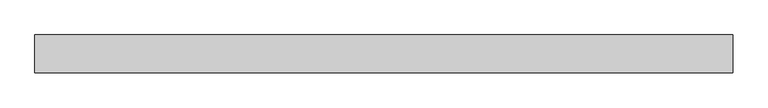
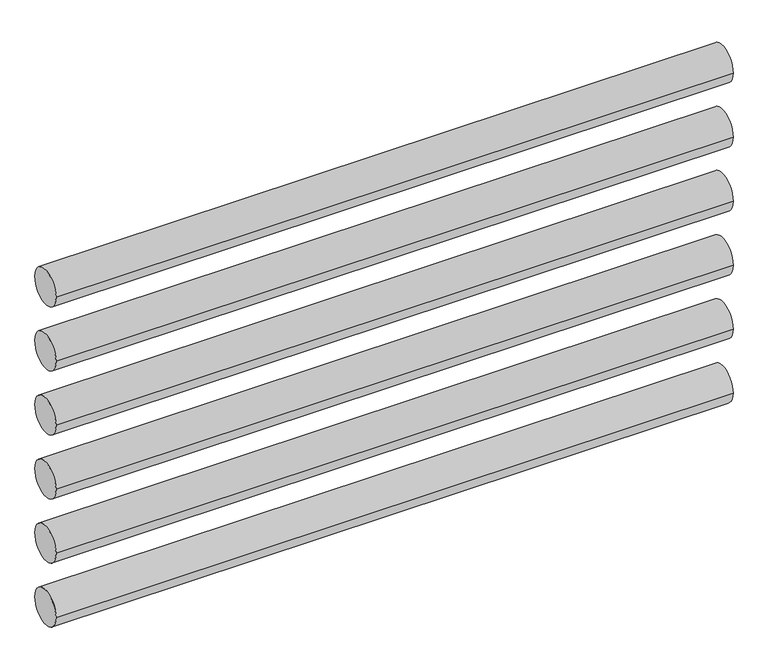
"""IFC4 building model written with IfcOpenShell, lengths in millimetres: proxy geometry, Газпремиум_Регистр : РГТ-1-108х3-2м-6."""

from ifc_helpers import new_model, si_unit, point, frame, frame_2d, origin, place, context, project, spatial, circle_curve, trimmed, segment, composite_curve, outline, extrude, source, transform, mapped, element, save


def mechanical_equipment_f739d76b(model_context):
    return source(origin(), model_context, "Body", "SweptSolid", [
        extrude(outline(composite_curve([segment(trimmed(circle_curve(frame_2d((0.0, 1054.0)), 54.0), [point((-54.0, 1054.0))], [point((54.0, 1054.0))], False, "CARTESIAN"), True, "CONTINUOUS"), segment(trimmed(circle_curve(frame_2d((0.0, 1054.0)), 54.0), [point((54.0, 1054.0))], [point((-54.0, 1054.0))], False, "CARTESIAN"), True, "CONTINUOUS")], self_intersect=False)), frame((-184.1719207, 0.0, 0.0), z_axis=(1.0, 0.0, 0.0), x_axis=(0.0, 1.0, 0.0)), (0.0, 0.0, 1.0), 2000.0),
        extrude(outline(composite_curve([segment(trimmed(circle_curve(frame_2d((0.0, 854.0)), 54.0), [point((-54.0, 854.0))], [point((54.0, 854.0))], False, "CARTESIAN"), True, "CONTINUOUS"), segment(trimmed(circle_curve(frame_2d((0.0, 854.0)), 54.0), [point((54.0, 854.0))], [point((-54.0, 854.0))], False, "CARTESIAN"), True, "CONTINUOUS")], self_intersect=False)), frame((-184.1719207, 0.0, 0.0), z_axis=(1.0, 0.0, 0.0), x_axis=(0.0, 1.0, 0.0)), (0.0, 0.0, 1.0), 2000.0),
        extrude(outline(composite_curve([segment(trimmed(circle_curve(frame_2d((0.0, 654.0)), 54.0), [point((-54.0, 654.0))], [point((54.0, 654.0))], False, "CARTESIAN"), True, "CONTINUOUS"), segment(trimmed(circle_curve(frame_2d((0.0, 654.0)), 54.0), [point((54.0, 654.0))], [point((-54.0, 654.0))], False, "CARTESIAN"), True, "CONTINUOUS")], self_intersect=False)), frame((-184.1719207, 0.0, 0.0), z_axis=(1.0, 0.0, 0.0), x_axis=(0.0, 1.0, 0.0)), (0.0, 0.0, 1.0), 2000.0),
        extrude(outline(composite_curve([segment(trimmed(circle_curve(frame_2d((0.0, 454.0)), 54.0), [point((-54.0, 454.0))], [point((54.0, 454.0))], False, "CARTESIAN"), True, "CONTINUOUS"), segment(trimmed(circle_curve(frame_2d((0.0, 454.0)), 54.0), [point((54.0, 454.0))], [point((-54.0, 454.0))], False, "CARTESIAN"), True, "CONTINUOUS")], self_intersect=False)), frame((-184.1719207, 0.0, 0.0), z_axis=(1.0, 0.0, 0.0), x_axis=(0.0, 1.0, 0.0)), (0.0, 0.0, 1.0), 2000.0),
        extrude(outline(composite_curve([segment(trimmed(circle_curve(frame_2d((0.0, 254.0)), 54.0), [point((-54.0, 254.0))], [point((54.0, 254.0))], False, "CARTESIAN"), True, "CONTINUOUS"), segment(trimmed(circle_curve(frame_2d((0.0, 254.0)), 54.0), [point((54.0, 254.0))], [point((-54.0, 254.0))], False, "CARTESIAN"), True, "CONTINUOUS")], self_intersect=False)), frame((-184.1719207, 0.0, 0.0), z_axis=(1.0, 0.0, 0.0), x_axis=(0.0, 1.0, 0.0)), (0.0, 0.0, 1.0), 2000.0),
        extrude(outline(composite_curve([segment(trimmed(circle_curve(frame_2d((0.0, 54.0)), 54.0), [point((-54.0, 54.0))], [point((54.0, 54.0))], False, "CARTESIAN"), True, "CONTINUOUS"), segment(trimmed(circle_curve(frame_2d((0.0, 54.0)), 54.0), [point((54.0, 54.0))], [point((-54.0, 54.0))], False, "CARTESIAN"), True, "CONTINUOUS")], self_intersect=False)), frame((-184.1719207, 0.0, 0.0), z_axis=(1.0, 0.0, 0.0), x_axis=(0.0, 1.0, 0.0)), (0.0, 0.0, 1.0), 2000.0),
    ])


if __name__ == "__main__":
    model = new_model("IFC4")
    model_context = context("Model", 3, world=origin())
    ifc_project = project(units=[si_unit("LENGTHUNIT", "METRE", prefix="MILLI")], contexts=[model_context])
    site = spatial("IfcSite", under=ifc_project)
    building = spatial("IfcBuilding", under=site)
    placement = place(None, origin())
    mechanical_equipment_shape = mechanical_equipment_f739d76b(model_context)
    element("IfcBuildingElementProxy", 1, Name="Газпремиум_Регистр : РГТ-1-108х3-2м-6", ObjectType="Газпремиум_Регистр : РГТ-1-108х3-2м-6", at=placement, inside=building, context=model_context, shape_type="MappedRepresentation", body=[
        mapped(mechanical_equipment_shape, transform((0.0, 0.0, 0.0), x_axis=(1.0, 0.0, 0.0), y_axis=(0.0, 1.0, 0.0), z_axis=(0.0, 0.0, 1.0))),
    ])
    save(model, "model.ifc")

# Revit data of these elements
# Type "Газпремиум_Регистр : РГТ-1-108х3-2м-6"
#   ADSK_Позиция = "390"
#   ADSK_Наименование = "Регистр однорядный из шести гладких труб 108х3 длиной 2 м, в комплекте с опорами"
#   ADSK_Марка = "РГТ-1-108х3-2м-6-ОП-О ТУ 4936-001-69441315-11"
#   ADSK_Код изделия = "2050868"
#   ADSK_Завод-изготовитель = "ООО ПКП \"ГазПремиум\", Россия, г.Саратов, ИНН 6452951387, кпп 645201001, gaz-premium@mail.ru"
#   ADSK_Единица измерения = "шт."
#   Расстояние между рядами = 200 mm
#   Радиус.регистра = 54 mm
#   Отступ.труб.подкл.от.осевой = 32.719 mm
#   Длина регистра = 2000 mm
#   Диаметр.труб.подкл. = 32 mm
#   Диаметр регистра = 108 mm
#   Высота = 1000 mm
#   ADSK_Масса = 116.29
#   ADSK_Количество = 1
#   Число рядов = 6
#   Соед.трубы = Грунтовка.красная
#   Регистр = Грунтовка.красная
#   Поддерж.арматура = Грунтовка.серая
#   Default Elevation = 0
# Element 1 (IfcBuildingElementProxy, "Газпремиум_Регистр : РГТ-1-108х3-2м-6")
#   Materials on its faces: "Грунтовка.красная"
# Materials
#   "Грунтовка.красная": class "Разное", colour RGB 255 0 0, transparency 0
#   "Грунтовка.серая": class "Разное", colour RGB 187 181 179, transparency 0
